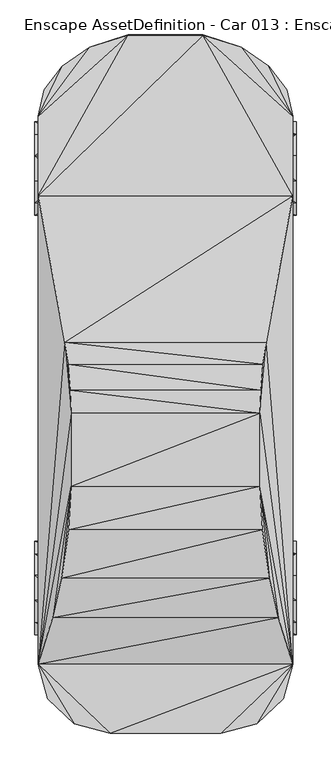
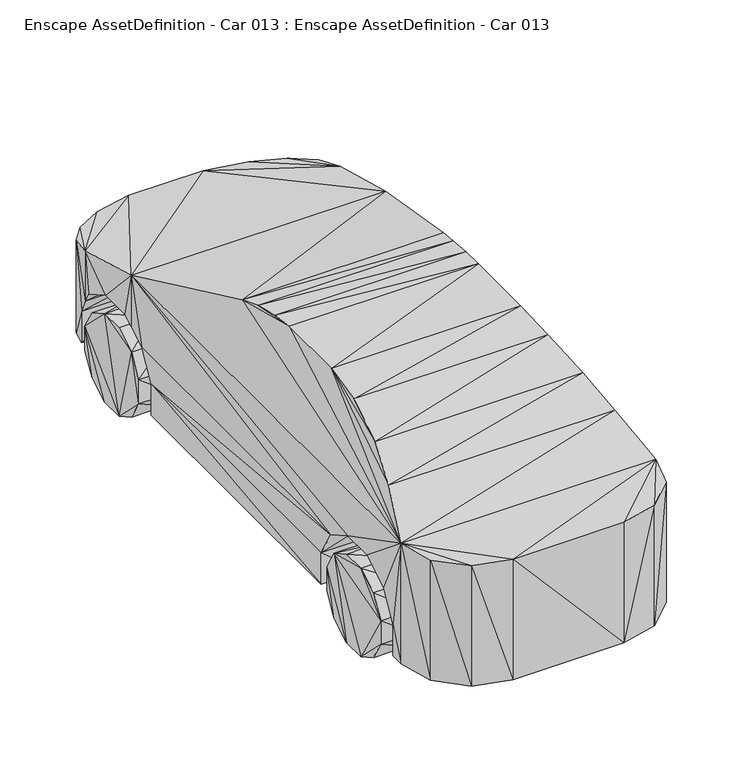
"""IFC4 building model written with IfcOpenShell, lengths in millimetres: geographic element geometry, Enscape AssetDefinition - Car 013 : Enscape AssetDefinition - Car 013."""

from ifc_helpers import new_model, si_unit, origin, place, context, project, spatial, faceted_brep, source, transform, mapped, element, save


def enscape_assetdefinition_car_013_enscape_assetdefinition_car_651e53f9(model_context):
    return source(origin(), model_context, "Body", "Brep", [
        faceted_brep([(559.9123836, -1227.6889086, 696.8670487), (559.9124432, -1042.8061485, 590.1246667), (812.2093678, -1227.6889086, 696.8670487), (559.9123836, -936.0638857, 405.241698), (812.2093678, -936.0638857, 405.241698), (812.2094274, -1042.8061485, 590.1246667), (559.9123836, -936.0639453, 192.5706565), (559.9123836, -1441.1734343, 696.8669295), (812.2093678, -936.0639453, 192.5706565), (559.9123836, -1732.7986956, 192.5706565), (559.9123836, 940.2685761, 192.5706565), (-559.9123836, -936.0639453, 192.5706565), (812.2093678, 940.2685165, 405.241996), (812.2093678, 940.2685761, 192.5706565), (559.9123836, 940.2685165, 405.241996), (812.2093678, 1047.0108986, 590.1249647), (559.9123836, 1047.0108986, 590.1249647), (559.9123836, 1164.4049883, 657.9024792), (812.2093678, 1164.4049883, 657.9024792), (812.2094274, 1164.4049883, 1000.2167225), (812.2093081, 1231.8935394, 696.8670487), (559.912324, 1231.8935394, 696.8670487), (559.9123836, 1445.3780651, 696.8670487), (812.2094274, 1445.3780651, 696.8670487), (559.9123836, 1671.0397005, 519.4937587), (559.9123836, 1630.2611828, 590.1246667), (812.2094274, 1630.2611828, 590.1246667), (812.2093678, 1671.0397005, 860.5755568), (812.2093678, 1671.0397005, 519.4937587), (796.810627, 1737.0032072, 405.2417874), (773.1425166, 1838.3886814, 814.449966), (483.1784666, 2109.1644764, 739.8173809), (237.4432683, 2187.1418953, 718.3248997), (659.7662568, 1989.356041, 772.8395462), (773.1425166, 1838.3886814, 192.5706565), (659.766376, 1989.356041, 192.5706565), (483.178556, 2109.1647148, 192.5706565), (549.2969155, 1737.003088, 192.5706714), (796.8105674, 1737.003088, 192.5706714), (549.2969751, 1737.0032072, 405.2417874), (-559.9123836, 940.2685761, 192.5706565), (237.4432683, 2188.4474754, 192.5706565), (-237.4432683, 2188.4474754, 192.5706565), (-549.2969751, 1737.003088, 192.5706714), (-237.4432683, 2187.1418953, 718.3248997), (-483.178556, 2109.1647148, 192.5706565), (-812.2094274, 1164.4049883, 1000.2167225), (-483.1784666, 2109.1644764, 739.8173809), (-812.2093678, 1671.0397005, 860.5755568), (-659.766376, 1989.356041, 192.5706565), (-659.7662568, 1989.356041, 772.8395462), (-773.1425166, 1838.3886814, 192.5706565), (-773.1425166, 1838.3886814, 814.449966), (-796.810627, 1737.0032072, 405.2417874), (-796.8105674, 1737.003088, 192.5706714), (-812.2093678, 1671.0397005, 519.4937587), (-549.2969751, 1737.0032072, 405.2417874), (-559.9123836, 1671.0397005, 519.4937587), (-559.9123836, 1164.4049883, 657.9024792), (-559.9124432, 1445.3780651, 696.8670487), (-559.9124432, 1630.2611828, 590.1246667), (-812.2094274, 1630.2611828, 590.1246667), (-812.2094274, 1445.3780651, 696.8670487), (-812.2093081, 1231.8935394, 696.8670487), (-559.912324, 1231.8935394, 696.8670487), (-812.2093678, 1164.4049883, 657.9024792), (-812.2093678, 1047.0108986, 590.1249647), (-559.9123836, 1047.0108986, 590.1249647), (-812.2093678, 940.2685165, 405.241996), (-812.2094274, -1042.8061485, 590.1246667), (-559.9123836, 940.2685165, 405.241996), (-812.2093678, 940.2685761, 192.5706565), (-812.2093678, -936.0639453, 192.5706565), (-812.2093678, -936.0638857, 405.241698), (-559.9123836, -1042.8061485, 590.1246667), (-812.2093678, -1227.6889086, 696.8670487), (-559.9123836, -936.0638857, 405.241698), (-559.9123836, -1441.1734343, 696.8669295), (-559.9123836, -1732.7986956, 192.5706565), (-559.9123836, -1227.6889086, 696.8670487), (-812.2093678, -1441.1734343, 696.8669295), (-559.9123836, -1626.0564327, 590.1247859), (-812.2094274, -1626.0564327, 590.1247859), (-812.2093081, -1820.9619522, 1004.3013096), (-812.2093678, -1732.7985764, 405.241847), (-559.9123836, -1732.7985764, 405.241847), (-812.2093678, -1732.7986956, 192.5706565), (-812.2093678, -1820.9619522, 192.5706565), (-750.7910728, -2040.4741764, 192.5706565), (-750.7910728, -2040.4741764, 1004.3013096), (-582.9930902, -2201.1685371, 192.5706565), (353.7767828, -2259.986639, 192.5706565), (-353.7767828, -2259.986639, 192.5706565), (-582.9930902, -2201.1685371, 1004.3013096), (-353.7767828, -2259.986639, 1004.3013096), (812.2093081, -1820.9619522, 1004.3013096), (353.7767828, -2259.986639, 1004.3013096), (582.9930902, -2201.1685371, 1004.3013096), (582.9930902, -2201.1685371, 192.5706565), (750.7910728, -2040.4741764, 1004.3013096), (750.7910728, -2040.4741764, 192.5706565), (812.2093678, -1820.9619522, 192.5706565), (812.2093678, -1732.7985764, 405.241847), (812.2093678, -1732.7986956, 192.5706565), (559.9123836, -1732.7985764, 405.241847), (559.9124432, -1626.0564327, 590.1247859), (812.2094274, -1626.0564327, 590.1247859), (812.2093678, -1441.1734343, 696.8669295), (-642.3395276, 230.8107615, 1343.265295), (642.3395276, 230.8108211, 1343.265295), (-602.5201082, -221.186161, 1423.6798286), (721.0939527, -1525.2724886, 1186.5320206), (-602.5200486, -688.4683371, 1423.6798286), (-721.0939527, -1525.2724886, 1186.5320206), (602.5201082, -221.186161, 1423.6798286), (-622.4298477, 90.1517719, 1383.4725618), (-607.8549027, -75.290598, 1412.9062891), (-661.806941, -1272.3158598, 1305.1059246), (-618.4058785, -966.02422, 1391.9081688), (602.5200486, -688.4683371, 1423.6798286), (661.806941, -1272.3158598, 1305.1059246), (618.4058785, -966.0243392, 1391.9081688), (622.4298477, 90.1517794, 1383.4725618), (607.8549027, -75.2906129, 1412.9062891)], [[[0, 1, 2]], [[3, 4, 1]], [[2, 1, 5]], [[1, 4, 5]], [[1, 6, 3]], [[6, 1, 0]], [[0, 2, 7]], [[6, 0, 7]], [[6, 8, 3]], [[7, 9, 6]], [[6, 10, 8]], [[11, 10, 6]], [[11, 6, 9]], [[3, 8, 4]], [[12, 8, 13]], [[12, 4, 8]], [[8, 10, 13]], [[10, 12, 13]], [[14, 12, 10]], [[14, 15, 12]], [[5, 12, 15]], [[12, 5, 4]], [[16, 15, 14]], [[17, 16, 14]], [[17, 14, 10]], [[16, 18, 15]], [[15, 18, 19]], [[5, 15, 19]], [[17, 18, 16]], [[17, 20, 18]], [[20, 19, 18]], [[21, 20, 17]], [[21, 22, 20]], [[20, 22, 23]], [[23, 19, 20]], [[17, 22, 21]], [[17, 24, 22]], [[17, 10, 24]], [[25, 26, 22]], [[22, 26, 23]], [[22, 24, 25]], [[27, 23, 26]], [[27, 19, 23]], [[25, 28, 26]], [[27, 26, 28]], [[24, 28, 25]], [[24, 29, 28]], [[28, 30, 27]], [[28, 29, 30]], [[27, 31, 32]], [[32, 19, 27]], [[33, 27, 30]], [[27, 33, 31]], [[34, 33, 30]], [[29, 34, 30]], [[35, 33, 34]], [[35, 31, 33]], [[36, 31, 35]], [[36, 32, 31]], [[37, 35, 34]], [[37, 36, 35]], [[34, 29, 38]], [[37, 34, 38]], [[37, 38, 39]], [[39, 38, 29]], [[39, 29, 24]], [[24, 37, 39]], [[24, 10, 37]], [[40, 37, 10]], [[40, 10, 11]], [[37, 41, 36]], [[37, 42, 41]], [[37, 43, 42]], [[37, 40, 43]], [[41, 32, 36]], [[42, 32, 41]], [[44, 32, 42]], [[45, 44, 42]], [[43, 45, 42]], [[46, 32, 44]], [[19, 32, 46]], [[47, 44, 45]], [[48, 44, 47]], [[44, 48, 46]], [[49, 47, 45]], [[43, 49, 45]], [[50, 47, 49]], [[48, 47, 50]], [[51, 50, 49]], [[43, 51, 49]], [[52, 50, 51]], [[48, 50, 52]], [[53, 52, 51]], [[53, 51, 54]], [[51, 43, 54]], [[52, 53, 55]], [[55, 48, 52]], [[53, 54, 56]], [[55, 53, 57]], [[57, 53, 56]], [[56, 54, 43]], [[57, 56, 43]], [[57, 43, 40]], [[57, 58, 59]], [[60, 55, 57]], [[57, 59, 60]], [[57, 40, 58]], [[61, 55, 60]], [[61, 48, 55]], [[61, 60, 62]], [[62, 60, 59]], [[62, 59, 63]], [[63, 59, 64]], [[59, 58, 64]], [[62, 46, 48]], [[46, 62, 63]], [[62, 48, 61]], [[65, 63, 58]], [[58, 63, 64]], [[46, 63, 65]], [[65, 58, 66]], [[66, 46, 65]], [[66, 67, 68]], [[66, 58, 67]], [[69, 46, 66]], [[69, 66, 68]], [[68, 67, 70]], [[58, 70, 67]], [[68, 70, 71]], [[72, 68, 71]], [[73, 68, 72]], [[69, 68, 73]], [[69, 73, 74]], [[69, 74, 75]], [[69, 75, 46]], [[72, 11, 73]], [[73, 11, 76]], [[74, 73, 76]], [[40, 72, 71]], [[40, 11, 72]], [[71, 70, 40]], [[58, 40, 70]], [[77, 11, 78]], [[11, 77, 79]], [[11, 79, 74]], [[11, 74, 76]], [[9, 78, 11]], [[75, 74, 79]], [[75, 79, 80]], [[80, 79, 77]], [[78, 81, 77]], [[81, 80, 77]], [[82, 80, 81]], [[83, 75, 80]], [[83, 80, 82]], [[82, 81, 84]], [[78, 85, 81]], [[84, 81, 85]], [[83, 82, 84]], [[84, 85, 86]], [[84, 86, 87]], [[84, 87, 83]], [[86, 85, 78]], [[78, 87, 86]], [[88, 83, 87]], [[78, 88, 87]], [[89, 83, 88]], [[90, 89, 88]], [[78, 90, 88]], [[91, 78, 9]], [[78, 91, 92]], [[78, 92, 90]], [[93, 89, 90]], [[92, 93, 90]], [[93, 83, 89]], [[94, 93, 92]], [[93, 94, 83]], [[92, 91, 94]], [[94, 95, 83]], [[95, 94, 96]], [[94, 91, 96]], [[96, 91, 97]], [[95, 96, 97]], [[97, 91, 98]], [[9, 98, 91]], [[95, 97, 99]], [[97, 98, 99]], [[99, 98, 100]], [[9, 100, 98]], [[99, 100, 95]], [[95, 100, 101]], [[100, 9, 101]], [[102, 95, 101]], [[102, 101, 103]], [[101, 9, 103]], [[104, 102, 9]], [[9, 102, 103]], [[9, 7, 105]], [[9, 105, 104]], [[104, 105, 102]], [[102, 105, 106]], [[106, 95, 102]], [[7, 107, 105]], [[105, 107, 106]], [[7, 2, 107]], [[2, 95, 107]], [[107, 95, 106]], [[2, 19, 95]], [[5, 19, 2]], [[46, 108, 19]], [[19, 108, 109]], [[109, 95, 19]], [[83, 108, 46]], [[75, 83, 46]], [[83, 110, 108]], [[95, 111, 83]], [[112, 83, 113]], [[83, 112, 110]], [[83, 111, 113]], [[110, 112, 114]], [[115, 110, 116]], [[115, 108, 110]], [[114, 116, 110]], [[112, 113, 117]], [[112, 117, 118]], [[114, 112, 119]], [[118, 119, 112]], [[111, 120, 113]], [[113, 120, 117]], [[120, 121, 117]], [[117, 121, 118]], [[121, 119, 118]], [[95, 114, 119]], [[120, 119, 121]], [[120, 111, 119]], [[119, 111, 95]], [[114, 95, 109]], [[109, 108, 122]], [[114, 109, 122]], [[122, 108, 115]], [[122, 115, 123]], [[114, 122, 123]], [[123, 116, 114]], [[123, 115, 116]]]),
        faceted_brep([(833.6846232, 1040.4093266, 218.5902148), (833.6846232, 1636.8623972, 378.4092367), (833.6846232, 1418.5454845, 596.7264175), (833.6846232, 1636.8623972, 218.5900956), (619.4707155, 1636.8623972, 378.4091771), (833.6846232, 1556.9529533, 516.8166757), (833.6846232, 1418.5452461, 0.2732367), (833.6846232, 1556.9527149, 80.1827237), (619.4706559, 1556.9527149, 80.1827237), (619.4706559, 1636.8623972, 218.5900956), (619.4706559, 1418.5452461, 0.2732367), (833.6846232, 1258.72612, 0.2732767), (619.4707155, 1258.72612, 0.2732767), (619.4707155, 1040.4093266, 218.5902148), (619.4707155, 1120.3188896, 516.8168545), (619.4707155, 1556.9529533, 516.8166757), (619.4707155, 1418.5454845, 596.7264175), (833.6846232, 1258.7262392, 596.7264175), (619.4707155, 1258.7262392, 596.7264175), (833.6846232, 1120.3188896, 516.8168545), (833.6846232, 1040.4092073, 378.4093857), (619.4707155, 1040.4092073, 378.4093857), (833.6846232, 1120.3187704, 80.1828578), (619.4707155, 1120.3187704, 80.1828578)], [[[0, 1, 2]], [[1, 3, 4]], [[1, 4, 5]], [[1, 6, 7]], [[1, 0, 6]], [[1, 7, 3]], [[2, 1, 5]], [[7, 8, 3]], [[3, 8, 9]], [[4, 3, 9]], [[6, 10, 7]], [[7, 10, 8]], [[11, 12, 6]], [[0, 11, 6]], [[6, 12, 10]], [[4, 8, 10]], [[13, 10, 12]], [[13, 4, 10]], [[8, 4, 9]], [[4, 13, 14]], [[14, 15, 4]], [[5, 4, 15]], [[14, 16, 15]], [[16, 5, 15]], [[2, 16, 17]], [[2, 5, 16]], [[16, 14, 18]], [[17, 16, 18]], [[17, 18, 19]], [[19, 2, 17]], [[0, 2, 19]], [[19, 14, 20]], [[0, 19, 20]], [[19, 18, 14]], [[20, 21, 0]], [[0, 13, 22]], [[11, 0, 22]], [[0, 21, 13]], [[20, 14, 21]], [[14, 13, 21]], [[13, 12, 23]], [[22, 13, 23]], [[22, 23, 11]], [[11, 23, 12]]]),
        faceted_brep([(833.6845636, -1414.3407345, 0.2731367), (833.6845636, -1116.114378, 516.8165565), (833.6845636, -1414.3407345, 596.7262387), (833.6845636, -1254.5218468, 596.7262387), (619.4706559, -1254.5218468, 596.7262387), (833.6845636, -1036.2046957, 378.4091175), (619.4705963, -1036.2046957, 378.4091175), (833.6845636, -1254.5218468, 0.2730867), (833.6845636, -1116.114378, 80.182597), (619.4705963, -1116.114378, 516.8165565), (619.4706559, -1414.3407345, 596.7262387), (619.4705963, -1414.3407345, 0.2731367), (619.4706559, -1632.6578856, 378.4092367), (833.6845636, -1552.7484417, 516.8166757), (619.4706559, -1552.7484417, 516.8166757), (833.6845636, -1632.6578856, 378.4092367), (833.6845636, -1632.6578856, 218.5900956), (619.4706559, -1632.6578856, 218.5900956), (833.6845636, -1552.7484417, 80.1827013), (619.4705963, -1552.7484417, 80.1827013), (619.4705963, -1254.5218468, 0.2730867), (619.4705963, -1116.114378, 80.182597), (833.6845636, -1036.2046957, 218.5899764), (619.4705963, -1036.2046957, 218.5899764)], [[[0, 1, 2]], [[3, 1, 4]], [[5, 6, 1]], [[1, 3, 2]], [[1, 0, 7]], [[1, 7, 8]], [[8, 5, 1]], [[4, 1, 9]], [[1, 6, 9]], [[3, 4, 2]], [[9, 10, 4]], [[2, 4, 10]], [[11, 9, 6]], [[9, 11, 12]], [[12, 10, 9]], [[2, 10, 13]], [[12, 14, 10]], [[13, 10, 14]], [[15, 12, 16]], [[11, 17, 12]], [[16, 12, 17]], [[15, 14, 12]], [[13, 14, 15]], [[15, 2, 13]], [[0, 2, 15]], [[16, 0, 15]], [[16, 17, 18]], [[0, 16, 18]], [[17, 11, 19]], [[18, 17, 19]], [[18, 19, 0]], [[0, 11, 7]], [[0, 19, 11]], [[7, 20, 8]], [[7, 11, 20]], [[11, 21, 20]], [[8, 20, 21]], [[8, 21, 22]], [[5, 8, 22]], [[11, 6, 21]], [[21, 6, 23]], [[22, 21, 23]], [[22, 23, 5]], [[5, 23, 6]]]),
        faceted_brep([(-619.4706559, 1418.5454845, 596.7263579), (-619.4706559, 1040.4093266, 218.5902148), (-619.4706559, 1556.9527149, 80.1827237), (-619.4706559, 1040.4092073, 378.4093857), (-833.6845636, 1040.4092073, 378.4093857), (-833.6845636, 1040.4093266, 218.5902148), (-619.4706559, 1120.3187704, 80.1828355), (-619.4706559, 1120.3188896, 516.8167949), (-619.4706559, 1258.72612, 0.2732767), (-833.6845636, 1120.3188896, 516.8168545), (-833.6845636, 1258.7262392, 0.2732867), (-833.6845636, 1120.3187704, 80.1828578), (-619.4706559, 1418.5452461, 0.2732167), (-833.6845636, 1636.8623972, 378.4092367), (-833.6845636, 1418.5452461, 0.2732367), (-833.6845636, 1418.5454845, 596.7264175), (-833.6845636, 1556.9527149, 80.1827386), (-619.4706559, 1636.8623972, 218.5900956), (-619.4706559, 1636.8623972, 378.4092367), (-619.4706559, 1556.9529533, 516.8166757), (-833.6845636, 1636.8623972, 218.5900956), (-833.6845636, 1556.9529533, 516.8166757), (-619.4706559, 1258.7262392, 596.7263579), (-833.6845636, 1258.7262392, 596.7264175)], [[[0, 1, 2]], [[3, 4, 1]], [[1, 5, 6]], [[1, 7, 3]], [[8, 1, 6]], [[1, 0, 7]], [[2, 1, 8]], [[1, 4, 5]], [[3, 7, 4]], [[9, 5, 4]], [[4, 7, 9]], [[9, 10, 5]], [[5, 10, 11]], [[6, 5, 11]], [[6, 11, 8]], [[8, 10, 12]], [[2, 8, 12]], [[8, 11, 10]], [[13, 14, 10]], [[10, 9, 15]], [[10, 15, 13]], [[12, 10, 14]], [[12, 14, 2]], [[13, 16, 14]], [[2, 14, 16]], [[2, 16, 17]], [[18, 2, 17]], [[2, 18, 19]], [[2, 19, 0]], [[16, 13, 20]], [[17, 16, 20]], [[17, 20, 18]], [[18, 13, 19]], [[18, 20, 13]], [[0, 19, 15]], [[19, 13, 21]], [[15, 19, 21]], [[13, 15, 21]], [[0, 15, 22]], [[15, 9, 23]], [[22, 15, 23]], [[7, 0, 22]], [[7, 22, 9]], [[9, 22, 23]]]),
        faceted_brep([(-619.4706559, -1116.114378, 516.8165565), (-619.4706559, -1632.6578856, 218.5900956), (-619.4706559, -1414.3407345, 0.2731167), (-619.4706559, -1632.6578856, 378.4092367), (-833.6845636, -1632.6578856, 378.4092367), (-833.6845636, -1632.6578856, 218.5900956), (-619.4706559, -1552.7484417, 80.1826864), (-619.4706559, -1254.5218468, 596.7262387), (-619.4706559, -1552.7484417, 516.8166757), (-833.6845636, -1552.7484417, 516.8166757), (-619.4706559, -1414.3407345, 596.7262387), (-833.6845636, -1116.114378, 516.8165565), (-833.6845636, -1254.5218468, 596.7262387), (-833.6845636, -1414.3407345, 596.7262387), (-833.6845636, -1254.5218468, 0.2730967), (-833.6845636, -1036.2046957, 378.4091175), (-833.6845636, -1414.3407345, 0.2731367), (-833.6845636, -1116.114378, 80.182597), (-619.4706559, -1254.5218468, 0.2730867), (-619.4706559, -1116.114378, 80.1825896), (-619.4706559, -1036.2046957, 218.5899764), (-833.6845636, -1036.2046957, 218.5899764), (-619.4706559, -1036.2046957, 378.4091175), (-833.6845636, -1552.7484417, 80.1827013)], [[[0, 1, 2]], [[3, 4, 1]], [[1, 5, 6]], [[7, 3, 1]], [[2, 1, 6]], [[1, 0, 7]], [[1, 4, 5]], [[8, 9, 3]], [[3, 7, 10]], [[3, 10, 8]], [[3, 9, 4]], [[0, 11, 7]], [[7, 12, 10]], [[7, 11, 12]], [[10, 13, 8]], [[10, 12, 13]], [[8, 13, 9]], [[4, 9, 13]], [[4, 13, 11]], [[11, 13, 12]], [[14, 11, 15]], [[11, 14, 16]], [[11, 16, 4]], [[0, 15, 11]], [[15, 17, 14]], [[18, 16, 14]], [[17, 18, 14]], [[19, 18, 17]], [[19, 17, 20]], [[17, 15, 21]], [[20, 17, 21]], [[2, 16, 18]], [[19, 2, 18]], [[22, 19, 20]], [[19, 22, 0]], [[2, 19, 0]], [[22, 15, 0]], [[20, 21, 22]], [[22, 21, 15]], [[6, 23, 2]], [[2, 23, 16]], [[5, 16, 23]], [[6, 5, 23]], [[16, 5, 4]]]),
    ])


if __name__ == "__main__":
    model = new_model("IFC4")
    model_context = context("Model", 3, world=origin())
    ifc_project = project(units=[si_unit("LENGTHUNIT", "METRE", prefix="MILLI")], contexts=[model_context])
    site = spatial("IfcSite", under=ifc_project)
    building = spatial("IfcBuilding", under=site)
    placement = place(None, origin())
    enscape_assetdefinition_car_013_enscape_assetdefinition_car_shape = enscape_assetdefinition_car_013_enscape_assetdefinition_car_651e53f9(model_context)
    element("IfcGeographicElement", 1, ObjectType="Enscape AssetDefinition - Car 013 : Enscape AssetDefinition - Car 013", at=placement, inside=building, context=model_context, shape_type="MappedRepresentation", body=[
        mapped(enscape_assetdefinition_car_013_enscape_assetdefinition_car_shape, transform((0.0, 0.0, 0.0), x_axis=(1.0, 0.0, 0.0), y_axis=(0.0, 1.0, 0.0), z_axis=(0.0, 0.0, 1.0))),
    ])
    save(model, "model.ifc")

# Revit data of these elements
# Type "Enscape AssetDefinition - Car 013 : Enscape AssetDefinition - Car 013"
#   EnscapeAssetSource = "REMOTE"
#   EnscapeAssetId = "6544ff70-f4b2-4605-b29f-758e2e405712"
#   Height = 1.42368 m
#   EnscapeNativeAssetHeight = 1.42368 m
#   Default Elevation = 0
